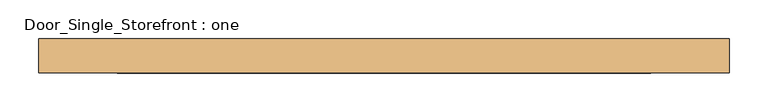
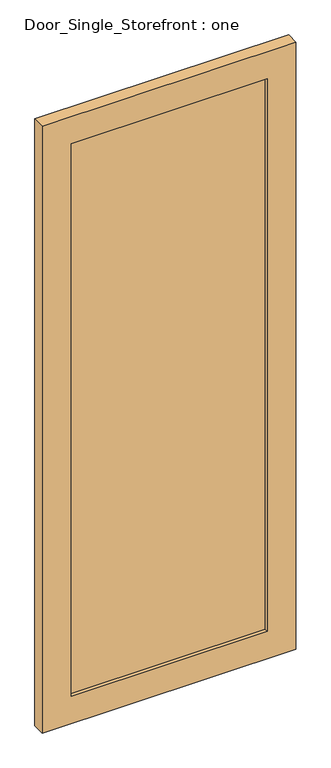
"""IFC4 building model written with IfcOpenShell, lengths in millimetres: door geometry, Door_Single_Storefront : one."""

from ifc_helpers import new_model, si_unit, frame, origin, place, context, project, spatial, polyline, outline, extrude, source, transform, mapped, element, save


def door_single_storefront_one_d6f978d6(model_context):
    return source(origin(), model_context, "Body", "SweptSolid", [
        extrude(outline(polyline([(345.28125, -19.05), (345.28125, -38.1), (-345.28125, -38.1), (-345.28125, -19.05), (345.28125, -19.05)])), frame((0.0, 0.0, 101.6), z_axis=(0.0, 0.0, 1.0), x_axis=(1.0, 0.0, 0.0)), (0.0, 0.0, 1.0), 2057.4),
        extrude(outline(polyline([(2260.6, -446.88125), (0.0, -446.88125), (0.0, 446.88125), (2260.6, 446.88125), (2260.6, -446.88125)]), holes=[polyline([(101.6, 345.28125), (101.6, -345.28125), (2159.0, -345.28125), (2159.0, 345.28125), (101.6, 345.28125)])]), frame((0.0, -50.8, 0.0), z_axis=(0.0, 1.0, 0.0), x_axis=(0.0, 0.0, 1.0)), (0.0, 0.0, 1.0), 44.45),
    ])


if __name__ == "__main__":
    model = new_model("IFC4")
    model_context = context("Model", 3, world=origin())
    ifc_project = project(units=[si_unit("LENGTHUNIT", "METRE", prefix="MILLI")], contexts=[model_context])
    site = spatial("IfcSite", under=ifc_project)
    building = spatial("IfcBuilding", under=site)
    placement = place(None, origin())
    door_single_storefront_one_shape = door_single_storefront_one_d6f978d6(model_context)
    element("IfcDoor", 1, ObjectType="Door_Single_Storefront : one", at=placement, inside=building, context=model_context, shape_type="MappedRepresentation", body=[
        mapped(door_single_storefront_one_shape, transform((0.0, 0.0, 0.0), x_axis=(1.0, 0.0, 0.0), y_axis=(0.0, 1.0, 0.0), z_axis=(0.0, 0.0, 1.0))),
    ])
    save(model, "model.ifc")

# Revit data of these elements
# Type "Door_Single_Storefront : one"
#   Type Mark = "27"
#   Analytic Construction = "<None>"
#   Stile_Width = 0' - 4"
#   Door_Thickness = 0' - 1 3/4"
#   Door_Offset = 0' - 2"
#   Glass_Material = Glass
#   Frame_Material = Aluminum
#   Function = (empty or 0)
# Element 1 (IfcDoor, "Door_Single_Storefront : one")
#   Materials on its faces: "Aluminum", "Glass"
# Materials
#   "Glass": class "Glass", colour RGB 0 128 192, transparency 0.75, Description = "Soda Lime Glass", Cost = 0
#   "Aluminum": class "Metal", colour RGB 247 247 247, transparency 0, Description = "Aluminum 6061", Cost = 0
